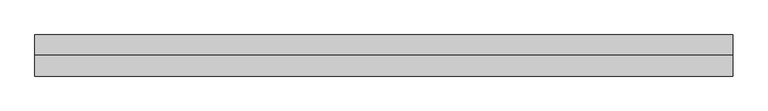
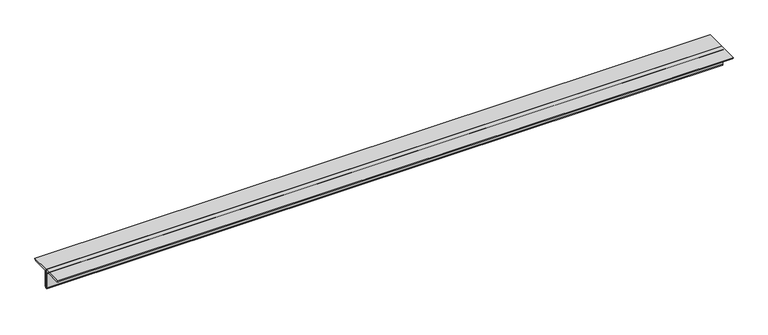
"""IFC4 building model written with IfcOpenShell, lengths in millimetres: member geometry, 0123_Steel Framing_2Ls-KSD3502 : H_SB_AR_S03_2Ls-130x130x12_HBR1."""

from ifc_helpers import new_model, si_unit, point, frame, frame_2d, origin, place, context, project, spatial, polyline, circle_curve, trimmed, segment, composite_curve, outline, extrude, source, transform, mapped, element, save


def member_bcbd117d(model_context):
    return source(origin(), model_context, "Body", "SweptSolid", [
        extrude(outline(composite_curve([segment(polyline([(0.0, 36.4), (0.0, -93.6)]), True, "CONTINUOUS"), segment(trimmed(circle_curve(frame_2d((0.0, -81.6)), 12.0), [point((0.0, -93.6))], [point((-12.0, -81.6))], False, "CARTESIAN"), True, "CONTINUOUS"), segment(polyline([(-12.0, -81.6), (-12.0, 12.4)]), True, "CONTINUOUS"), segment(trimmed(circle_curve(frame_2d((-24.0, 12.4)), 12.0), [point((-12.0, 12.4))], [point((-24.0, 24.4))], True, "CARTESIAN"), True, "CONTINUOUS"), segment(polyline([(-24.0, 24.4), (-118.0, 24.4)]), True, "CONTINUOUS"), segment(trimmed(circle_curve(frame_2d((-118.0, 36.4)), 12.0), [point((-118.0, 24.4))], [point((-130.0, 36.4))], False, "CARTESIAN"), True, "CONTINUOUS"), segment(polyline([(-130.0, 36.4), (0.0, 36.4)]), True, "CONTINUOUS")], self_intersect=False)), frame((-2209.5676318, 0.0, 0.0), z_axis=(1.0, 0.0, 0.0), x_axis=(0.0, 1.0, 0.0)), (0.0, 0.0, 1.0), 4412.2019305),
        extrude(outline(composite_curve([segment(polyline([(0.0, 36.4), (130.0, 36.4)]), True, "CONTINUOUS"), segment(trimmed(circle_curve(frame_2d((118.0, 36.4)), 12.0), [point((130.0, 36.4))], [point((118.0, 24.4))], False, "CARTESIAN"), True, "CONTINUOUS"), segment(polyline([(118.0, 24.4), (24.0, 24.4)]), True, "CONTINUOUS"), segment(trimmed(circle_curve(frame_2d((24.0, 12.4)), 12.0), [point((24.0, 24.4))], [point((12.0, 12.4))], True, "CARTESIAN"), True, "CONTINUOUS"), segment(polyline([(12.0, 12.4), (12.0, -81.6)]), True, "CONTINUOUS"), segment(trimmed(circle_curve(frame_2d((0.0, -81.6)), 12.0), [point((12.0, -81.6))], [point((0.0, -93.6))], False, "CARTESIAN"), True, "CONTINUOUS"), segment(polyline([(0.0, -93.6), (0.0, 36.4)]), True, "CONTINUOUS")], self_intersect=False)), frame((-2209.5676318, 0.0, 0.0), z_axis=(1.0, 0.0, 0.0), x_axis=(0.0, 1.0, 0.0)), (0.0, 0.0, 1.0), 4412.2019305),
    ])


if __name__ == "__main__":
    model = new_model("IFC4")
    model_context = context("Model", 3, world=origin())
    ifc_project = project(units=[si_unit("LENGTHUNIT", "METRE", prefix="MILLI")], contexts=[model_context])
    site = spatial("IfcSite", under=ifc_project)
    building = spatial("IfcBuilding", under=site)
    placement = place(None, origin())
    member_shape = member_bcbd117d(model_context)
    element("IfcMember", 1, ObjectType="0123_Steel Framing_2Ls-KSD3502 : H_SB_AR_S03_2Ls-130x130x12_HBR1", at=placement, inside=building, context=model_context, shape_type="MappedRepresentation", body=[
        mapped(member_shape, transform((0.0, 0.0, 0.0), x_axis=(1.0, 0.0, 0.0), y_axis=(0.0, 1.0, 0.0), z_axis=(0.0, 0.0, 1.0))),
    ])
    save(model, "model.ifc")

# Revit data of these elements
# Type "0123_Steel Framing_2Ls-KSD3502 : H_SB_AR_S03_2Ls-130x130x12_HBR1"
#   Assembly Code = "B10"
#   Legs = "SLBB"
#   W = 8.97
#   Perimeter = 1.04 m²/m
#   Nominal Weight = 46.80 kgf/m
#   Length [instance default] = 1000 mm
#   Space = 0 mm
#   b = 130 mm
#   d = 130 mm
#   t = 12 mm
#   y = 36.4 mm
#   A = 0.005952 m²
#   Structural Material [instance default] = Steel ASTM A36
# Element 1 (IfcMember, "0123_Steel Framing_2Ls-KSD3502 : H_SB_AR_S03_2Ls-130x130x12_HBR1")
#   Structural Material = Steel, 45-345
#   Materials on its faces: "Steel, 45-345"
# Materials
#   "Steel ASTM A36": class "Metal", colour RGB 199 199 199, transparency 0, Description = "Structural steel, ASTM A36 Grade B, mill finish", Cost = 0
#   "Steel, 45-345": class "Metal", colour RGB 189 187 185, transparency 0, Description = "Steel 345 MPa", Cost = 0
